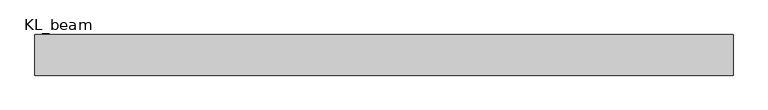
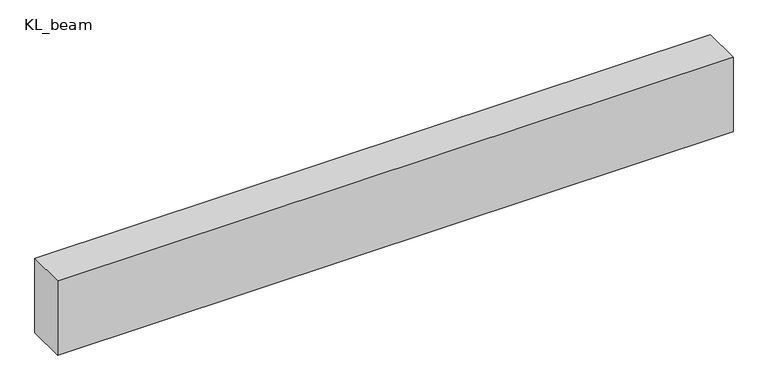
"""IFC4 building model written with IfcOpenShell, lengths in millimetres: beam geometry, 混凝土 - 矩形梁 : KL_beam."""

from ifc_helpers import new_model, si_unit, frame, origin, place, context, project, spatial, polyline, outline, extrude, source, transform, mapped, element, save


def kl_beam_04983839(model_context):
    return source(origin(), model_context, "Body", "SweptSolid", [
        extrude(outline(polyline([(3434.5, 200.0), (3434.5, -200.0), (-3434.5, -200.0), (-3434.5, 200.0), (3434.5, 200.0)])), frame((0.0, 0.0, -400.0), z_axis=(0.0, 0.0, 1.0), x_axis=(1.0, 0.0, 0.0)), (0.0, 0.0, 1.0), 800.0),
    ])


if __name__ == "__main__":
    model = new_model("IFC4")
    model_context = context("Model", 3, world=origin())
    ifc_project = project(units=[si_unit("LENGTHUNIT", "METRE", prefix="MILLI")], contexts=[model_context])
    site = spatial("IfcSite", under=ifc_project)
    building = spatial("IfcBuilding", under=site)
    placement = place(None, origin())
    kl_beam_shape = kl_beam_04983839(model_context)
    element("IfcBeam", 1, ObjectType="混凝土 - 矩形梁 : KL_beam", at=placement, inside=building, context=model_context, shape_type="MappedRepresentation", body=[
        mapped(kl_beam_shape, transform((0.0, 0.0, 0.0), x_axis=(1.0, 0.0, 0.0), y_axis=(0.0, 1.0, 0.0), z_axis=(0.0, 0.0, 1.0))),
    ])
    save(model, "model.ifc")

# Revit data of these elements
# Type "混凝土 - 矩形梁 : KL_beam"
#   Length [instance default] = 1524 mm
#   b = 400 mm
#   h = 800 mm
#   Structural Material [instance default] = 混凝土 - 现场浇注混凝土
#   Assembly Code = ""
# Element 1 (IfcBeam, "混凝土 - 矩形梁 : KL_beam")
#   Structural Material = none
# Materials
#   "混凝土 - 现场浇注混凝土": class "混凝土", colour RGB 192 192 192, transparency 0
